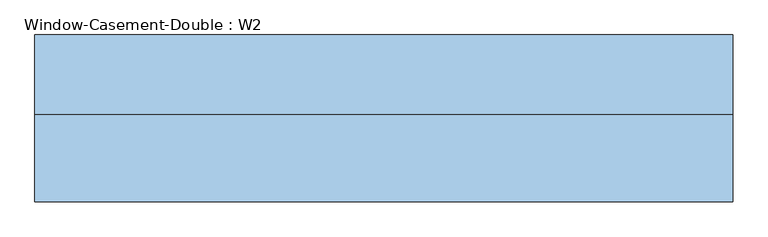
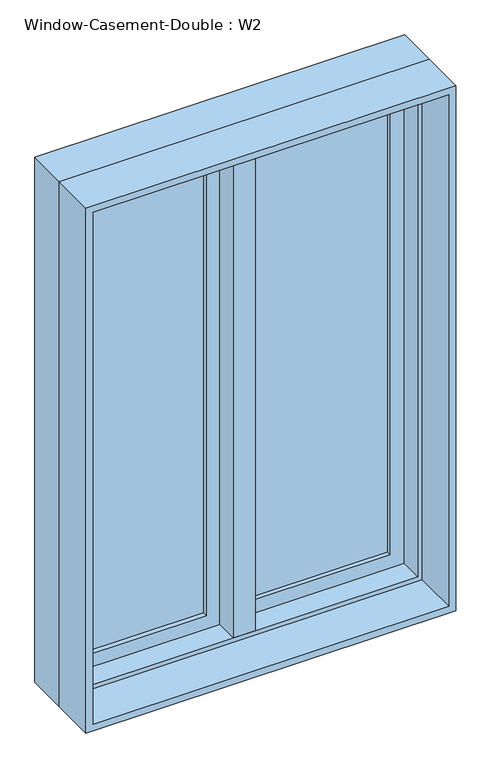
"""IFC4 building model written with IfcOpenShell, lengths in millimetres: window geometry, Window-Casement-Double : W2."""

from ifc_helpers import new_model, si_unit, frame, origin, place, context, project, spatial, polyline, outline, extrude, faceted_brep, source, transform, mapped, element, save


def window_casement_double_w2_23809e8b(model_context):
    return source(origin(), model_context, "Body", "SolidModel", [
        faceted_brep([(9.525, 129.05, 2401.7), (-9.525, 129.05, 2401.7), (-9.525, 78.25, 2401.7), (9.525, 78.25, 2401.7), (9.525, 129.05, 927.1), (9.525, 78.25, 927.1), (-9.525, 78.25, 927.1), (-9.525, 129.05, 927.1), (-9.525, 78.25, 946.15), (-9.525, 78.25, 2382.65), (-30.1625, 78.25, 946.15), (-30.1625, 78.25, 2382.65), (-30.1625, 14.75, 946.15), (-30.1625, 14.75, 2382.65), (30.1625, 14.75, 946.15), (30.1625, 14.75, 2382.65), (30.1625, 78.25, 946.15), (30.1625, 78.25, 2382.65), (9.525, 78.25, 946.15), (9.525, 78.25, 2382.65)], [[[0, 1, 2, 3]], [[4, 5, 6, 7]], [[1, 0, 4, 7]], [[2, 1, 7, 6, 8, 9]], [[9, 8, 10, 11]], [[11, 10, 12, 13]], [[13, 12, 14, 15]], [[15, 14, 16, 17]], [[17, 16, 18, 19]], [[0, 3, 19, 18, 5, 4]], [[18, 8, 6, 5]], [[9, 19, 3, 2]], [[8, 18, 16, 14, 12, 10]], [[19, 9, 11, 13, 15, 17]]]),
        extrude(outline(polyline([(-66.675, 110.0), (-66.675, 103.65), (-430.15, 103.65), (-430.15, 110.0), (-66.675, 110.0)])), frame((0.0, 0.0, 984.25), z_axis=(0.0, 0.0, 1.0), x_axis=(1.0, 0.0, 0.0)), (0.0, 0.0, 1.0), 1360.3),
        extrude(outline(polyline([(-430.15, 90.95), (-430.15, 97.3), (-66.675, 97.3), (-66.675, 90.95), (-430.15, 90.95)])), frame((0.0, 0.0, 984.25), z_axis=(0.0, 0.0, 1.0), x_axis=(1.0, 0.0, 0.0)), (0.0, 0.0, 1.0), 1360.3),
        extrude(outline(polyline([(430.15, 110.0), (430.15, 103.65), (66.675, 103.65), (66.675, 110.0), (430.15, 110.0)])), frame((0.0, 0.0, 984.25), z_axis=(0.0, 0.0, 1.0), x_axis=(1.0, 0.0, 0.0)), (0.0, 0.0, 1.0), 1360.3),
        extrude(outline(polyline([(66.675, 90.95), (66.675, 97.3), (430.15, 97.3), (430.15, 90.95), (66.675, 90.95)])), frame((0.0, 0.0, 984.25), z_axis=(0.0, 0.0, 1.0), x_axis=(1.0, 0.0, 0.0)), (0.0, 0.0, 1.0), 1360.3),
        extrude(outline(polyline([(2401.7, -487.3), (927.1, -487.3), (927.1, -9.525), (2401.7, -9.525), (2401.7, -487.3)]), holes=[polyline([(2344.55, -66.675), (984.25, -66.675), (984.25, -430.15), (2344.55, -430.15), (2344.55, -66.675)])]), frame((0.0, 78.25, 0.0), z_axis=(0.0, 1.0, 0.0), x_axis=(0.0, 0.0, 1.0)), (0.0, 0.0, 1.0), 44.45),
        extrude(outline(polyline([(927.1, 487.3), (2401.7, 487.3), (2401.7, 9.525), (927.1, 9.525), (927.1, 487.3)]), holes=[polyline([(984.25, 66.675), (2344.55, 66.675), (2344.55, 430.15), (984.25, 430.15), (984.25, 66.675)])]), frame((0.0, 78.25, 0.0), z_axis=(0.0, 1.0, 0.0), x_axis=(0.0, 0.0, 1.0)), (0.0, 0.0, 1.0), 44.45),
        extrude(outline(polyline([(2414.4, -500.0), (914.4, -500.0), (914.4, 500.0), (2414.4, 500.0), (2414.4, -500.0)]), holes=[polyline([(2395.35, 480.95), (933.45, 480.95), (933.45, -480.95), (2395.35, -480.95), (2395.35, 480.95)])]), frame((0.0, -110.0, 0.0), z_axis=(0.0, 1.0, 0.0), x_axis=(0.0, 0.0, 1.0)), (0.0, 0.0, 1.0), 124.75),
        faceted_brep([(468.25, 78.25, 2382.65), (468.25, 14.75, 2382.65), (-468.25, 14.75, 2382.65), (-468.25, 78.25, 2382.65), (487.3, 129.05, 2401.7), (487.3, 78.25, 2401.7), (-487.3, 78.25, 2401.7), (-487.3, 129.05, 2401.7), (500.0, 14.75, 2414.4), (500.0, 129.05, 2414.4), (-500.0, 129.05, 2414.4), (-500.0, 14.75, 2414.4), (-468.25, 14.75, 946.15), (-468.25, 78.25, 946.15), (-487.3, 78.25, 927.1), (-487.3, 129.05, 927.1), (-500.0, 129.05, 914.4), (-500.0, 14.75, 914.4), (468.25, 14.75, 946.15), (468.25, 78.25, 946.15), (487.3, 78.25, 927.1), (487.3, 129.05, 927.1), (500.0, 129.05, 914.4), (500.0, 14.75, 914.4)], [[[0, 1, 2, 3]], [[4, 5, 6, 7]], [[8, 9, 10, 11]], [[3, 2, 12, 13]], [[7, 6, 14, 15]], [[11, 10, 16, 17]], [[13, 12, 18, 19]], [[15, 14, 20, 21]], [[17, 16, 22, 23]], [[11, 17, 23, 8], [1, 18, 12, 2]], [[19, 18, 1, 0]], [[5, 20, 14, 6], [3, 13, 19, 0]], [[21, 20, 5, 4]], [[23, 22, 9, 8]], [[9, 22, 16, 10], [7, 15, 21, 4]]]),
    ])


if __name__ == "__main__":
    model = new_model("IFC4")
    model_context = context("Model", 3, world=origin())
    ifc_project = project(units=[si_unit("LENGTHUNIT", "METRE", prefix="MILLI")], contexts=[model_context])
    site = spatial("IfcSite", under=ifc_project)
    building = spatial("IfcBuilding", under=site)
    placement = place(None, origin())
    window_casement_double_w2_shape = window_casement_double_w2_23809e8b(model_context)
    element("IfcWindow", 1, ObjectType="Window-Casement-Double : W2", at=placement, inside=building, context=model_context, shape_type="MappedRepresentation", body=[
        mapped(window_casement_double_w2_shape, transform((0.0, 0.0, 0.0), x_axis=(1.0, 0.0, 0.0), y_axis=(0.0, 1.0, 0.0), z_axis=(0.0, 0.0, 1.0))),
    ])
    save(model, "model.ifc")

# Revit data of these elements
# Project information
#   Project Issue Date = "Issue Date"
#   Project Status = "Project Status"
#   Client Name = "Owner"
#   Project Address = "Enter address here"
#   Project Name = "Project Name"
#   Project Number = "0001"
# Type "Window-Casement-Double : W2"
#   Type Mark = "28"
#   Fire Rating = "0.5h"
#   Assembly Code = "B2020100"
#   Analytic Construction = "Double glazing - domestic"
#   Frame Extension [instance default] = 0.635 cm
#   Window Inset [instance default] = 0 cm
#   Wall Thickness [instance default] = 15.24 cm
#   Interior Wall Closure [instance default] = 5.715 cm
#   Half Width = 50 cm
#   Visual Light Transmittance = 0.81
#   Thermal Resistance (R) = 0.319569 (m²·K)/W
#   Solar Heat Gain Coefficient = 0.76
#   Rough Width = 101.27 cm
#   Rough Height = 151.27 cm
#   Height = 150 cm
#   Heat Transfer Coefficient (U) = 3.12929 W/(m²·K)
#   Exterior Wall Closure [instance default] = 3.175 cm
#   Extension Jamb [instance default] = 5.715 cm
#   Default Sill Height = 91.44 cm
#   Width = 100 cm
#   Muntin Visibility = yes
#   Interior Trim Visibility [instance default] = yes
#   Exterior Trim Visibility [instance default] = yes
#   Extension Jamb Visibility [instance default] = yes
#   Interior Trim Material = Wood - Stained
#   Muntin Pattern = Muntin Pattern_2x2 : Muntin Pattern_2x2
#   Interior Trim = Trim-Window-Interior-Flat : Picture Frame
#   Interior Frame Material = Wood - Stained
#   Glass Panel Material = Glass
#   Exterior Trim Material = Clad - White
#   Exterior Trim = Trim-Window-Exterior-Flat : with Sill
#   Exterior Frame Material = Clad - White
#   Wall Closure = (empty or 0)
# Element 1 (IfcWindow, "Window-Casement-Double : W2")
#   Wall Thickness = 22 cm
#   Extension Jamb = 12.475 cm
#   Materials on its faces: "Wood - Stained", "Glass", "Clad - White"
# Materials
#   "Wood - Stained": class "Wood", colour RGB 224 178 126, transparency 0, Cost = 0
#   "Glass": class "Glass", colour RGB 0 128 192, transparency 0.9, Description = "Soda Lime Glass", Cost = 0
#   "Clad - White": class "Wood", colour RGB 242 242 238, transparency 0, Cost = 0
